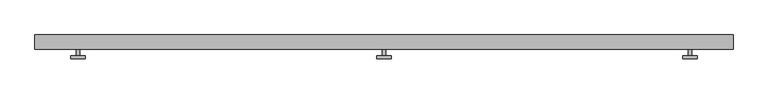
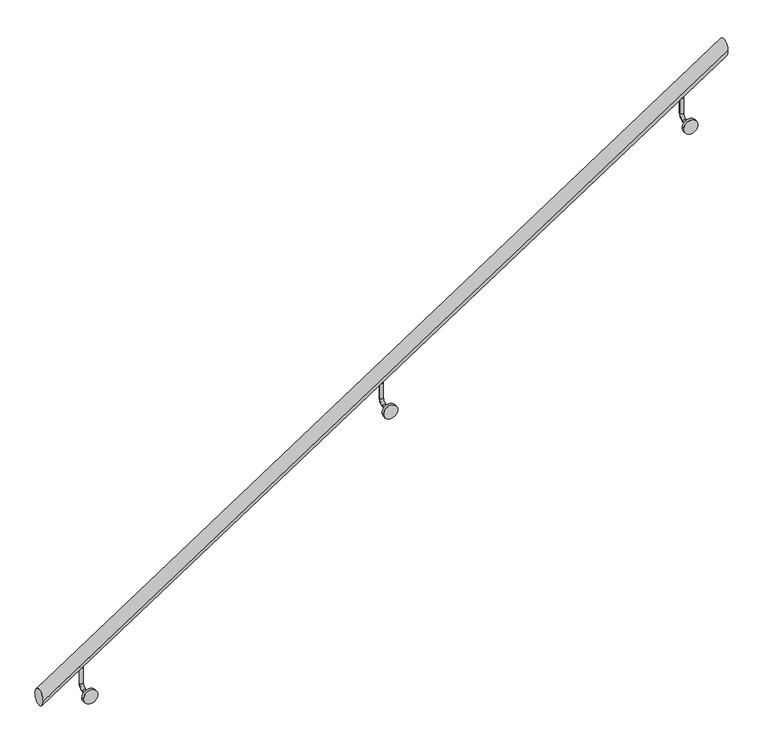
"""IFC4 building model written with IfcOpenShell, lengths in millimetres: railing geometry."""

from ifc_helpers import new_model, si_unit, point, frame, frame_2d, origin, place, context, project, spatial, circle_curve, ellipse_curve, trimmed, segment, composite_curve, outline, extrude, source, transform, mapped, element, save
from ifc_brep_helpers import plane_surface, cylinder_surface, revolved_surface, advanced_brep


def railing_45cfc386(model_context):
    return source(origin(), model_context, "Body", "SolidModel", [
        advanced_brep(
        [(-50271.1127262, 15484.3574868, 2840.3133544), (-50271.1127262, 15434.3574868, 2840.3133544), (-47841.1127262, 15484.3574868, 4430.3133544), (-47841.1127262, 15434.3574868, 4430.3133544)],
        [
            (0, 1, ellipse_curve(frame((-50271.1127262, 15459.3574868, 2840.3133544), z_axis=(-1.0, 0.0, 0.0), x_axis=(0.0, 0.0, -1.0)), 29.8761606, 25.0)),
            (1, 0, ellipse_curve(frame((-50271.1127262, 15459.3574868, 2840.3133544), z_axis=(-1.0, 0.0, 0.0), x_axis=(0.0, 0.0, -1.0)), 29.8761606, 25.0)),
            (2, 3, ellipse_curve(frame((-47841.1127262, 15459.3574868, 4430.3133544), z_axis=(1.0, 0.0, 0.0), x_axis=(0.0, 0.0, -1.0)), 29.8761606, 25.0)),
            (3, 2, ellipse_curve(frame((-47841.1127262, 15459.3574868, 4430.3133544), z_axis=(1.0, 0.0, 0.0), x_axis=(0.0, 0.0, -1.0)), 29.8761606, 25.0)),
            (0, 2),
            (3, 1),
        ],
        [
            plane_surface(frame((-50271.1127262, 15459.3574868, 2870.189515), z_axis=(-1.0, 0.0, 0.0), x_axis=(0.0, 1.0, 0.0))),
            plane_surface(frame((-47841.1127262, 15459.3574868, 4460.189515), z_axis=(1.0, 0.0, 0.0), x_axis=(0.0, 1.0, 0.0))),
            cylinder_surface(frame((-50257.4245344, 15459.3574868, 2849.2698256), z_axis=(-0.8367875758947572, 0.0, -0.547527673116324), x_axis=(0.0, -1.0, 0.0)), 25.0),
        ],
        [
            (0, [[1, 2]]),
            (1, [[3, 4]]),
            (2, [[-1, 5, -4, 6]]),
            (2, [[-2, -6, -3, -5]]),
        ],
    ),
        advanced_brep(
        [(-49062.4627262, 15459.3574868, 3596.139515), (-49049.7627262, 15459.3574868, 3596.139515), (-49062.4627262, 15459.3574868, 3538.989515), (-49049.7627262, 15459.3574868, 3538.989515), (-49049.7627262, 15440.3074868, 3519.939515), (-49062.4627262, 15440.3074868, 3519.939515), (-49062.4627262, 15411.7324868, 3519.939515), (-49049.7627262, 15411.7324868, 3519.939515)],
        [
            (0, 1, circle_curve(frame((-49056.1127262, 15459.3574868, 3596.139515), z_axis=(0.0, 0.0, 1.0), x_axis=(1.0, 0.0, 0.0)), 6.35)),
            (1, 0, circle_curve(frame((-49056.1127262, 15459.3574868, 3596.139515), z_axis=(0.0, 0.0, 1.0), x_axis=(1.0, 0.0, 0.0)), 6.35)),
            (0, 2),
            (2, 3, circle_curve(frame((-49056.1127262, 15459.3574868, 3538.989515), z_axis=(0.0, 0.0, 1.0), x_axis=(1.0, 0.0, 0.0)), 6.35)),
            (3, 1),
            (3, 2, circle_curve(frame((-49056.1127262, 15459.3574868, 3538.989515), z_axis=(0.0, 0.0, 1.0), x_axis=(1.0, 0.0, 0.0)), 6.35)),
            (4, 3, circle_curve(frame((-49049.7627262, 15440.3074868, 3538.989515), z_axis=(1.0, 0.0, 0.0), x_axis=(0.0, 1.0, 0.0)), 19.05)),
            (2, 5, circle_curve(frame((-49062.4627262, 15440.3074868, 3538.989515), z_axis=(-1.0, 0.0, 0.0), x_axis=(0.0, 1.0, 0.0)), 19.05)),
            (5, 4, circle_curve(frame((-49056.1127262, 15440.3074868, 3519.939515), z_axis=(0.0, 1.0, 0.0), x_axis=(1.0, 0.0, 0.0)), 6.35)),
            (4, 5, circle_curve(frame((-49056.1127262, 15440.3074868, 3519.939515), z_axis=(0.0, 1.0, 0.0), x_axis=(1.0, 0.0, 0.0)), 6.35)),
            (6, 7, circle_curve(frame((-49056.1127262, 15411.7324868, 3519.939515), z_axis=(0.0, -1.0, 0.0), x_axis=(1.0, 0.0, 0.0)), 6.35)),
            (7, 6, circle_curve(frame((-49056.1127262, 15411.7324868, 3519.939515), z_axis=(0.0, -1.0, 0.0), x_axis=(1.0, 0.0, 0.0)), 6.35)),
            (5, 6),
            (7, 4),
        ],
        [
            plane_surface(frame((-49049.7627262, 15459.3574868, 3596.139515), z_axis=(0.0, 0.0, 1.0), x_axis=(0.0, -1.0, 0.0))),
            cylinder_surface(frame((-49056.1127262, 15459.3574868, 3596.139515), z_axis=(0.0, 0.0, 1.0), x_axis=(1.0, 0.0, 0.0)), 6.35),
            revolved_surface(trimmed(ellipse_curve(frame((-49056.1127262, 15459.3574868, 3538.989515), z_axis=(0.0, 0.0, 1.0), x_axis=(1.0, 0.0, 0.0)), 6.35, 6.35), [point((-49062.4627262, 15459.3574868, 3538.989515))], [point((-49049.7627262, 15459.3574868, 3538.989515))], True, "CARTESIAN"), (-49056.1127262, 15440.3074868, 3538.989515), (-1.0, 0.0, 0.0)),
            revolved_surface(trimmed(ellipse_curve(frame((-49056.1127262, 15459.3574868, 3538.989515), z_axis=(0.0, 0.0, 1.0), x_axis=(1.0, 0.0, 0.0)), 6.35, 6.35), [point((-49049.7627262, 15459.3574868, 3538.989515))], [point((-49062.4627262, 15459.3574868, 3538.989515))], True, "CARTESIAN"), (-49056.1127262, 15440.3074868, 3538.989515), (-1.0, 0.0, 0.0)),
            plane_surface(frame((-49056.1127262, 15411.7324868, 3513.589515), z_axis=(0.0, -1.0, 0.0), x_axis=(1.0, 0.0, 0.0))),
            cylinder_surface(frame((-49056.1127262, 15440.3074868, 3519.939515), z_axis=(0.0, 1.0, 0.0), x_axis=(1.0, 0.0, 0.0)), 6.35),
        ],
        [
            (0, [[1, 2]]),
            (1, [[-1, 3, 4, 5]]),
            (1, [[-2, -5, 6, -3]]),
            (2, [[7, -4, 8, 9]]),
            (3, [[-8, -6, -7, 10]]),
            (4, [[11, 12]]),
            (5, [[-9, 13, -12, 14]]),
            (5, [[-10, -14, -11, -13]]),
        ],
    ),
        extrude(outline(composite_curve([segment(trimmed(circle_curve(frame_2d((3519.939515, -49056.1127262)), 25.4), [point((3519.939515, -49030.7127262))], [point((3519.939515, -49081.5127262))], False, "CARTESIAN"), True, "CONTINUOUS"), segment(trimmed(circle_curve(frame_2d((3519.939515, -49056.1127262)), 25.4), [point((3519.939515, -49081.5127262))], [point((3519.939515, -49030.7127262))], False, "CARTESIAN"), True, "CONTINUOUS")], self_intersect=False)), frame((0.0, 15402.2074868, 0.0), z_axis=(0.0, 1.0, 0.0), x_axis=(0.0, 0.0, 1.0)), (0.0, 0.0, 1.0), 9.525),
        advanced_brep(
        [(-47997.4627262, 15459.3574868, 4292.9913669), (-47984.7627262, 15459.3574868, 4292.9913669), (-47997.4627262, 15459.3574868, 4235.8413669), (-47984.7627262, 15459.3574868, 4235.8413669), (-47984.7627262, 15440.3074868, 4216.7913669), (-47997.4627262, 15440.3074868, 4216.7913669), (-47997.4627262, 15411.7324868, 4216.7913669), (-47984.7627262, 15411.7324868, 4216.7913669)],
        [
            (0, 1, circle_curve(frame((-47991.1127262, 15459.3574868, 4292.9913669), z_axis=(0.0, 0.0, 1.0), x_axis=(1.0, 0.0, 0.0)), 6.35)),
            (1, 0, circle_curve(frame((-47991.1127262, 15459.3574868, 4292.9913669), z_axis=(0.0, 0.0, 1.0), x_axis=(1.0, 0.0, 0.0)), 6.35)),
            (0, 2),
            (2, 3, circle_curve(frame((-47991.1127262, 15459.3574868, 4235.8413669), z_axis=(0.0, 0.0, 1.0), x_axis=(1.0, 0.0, 0.0)), 6.35)),
            (3, 1),
            (3, 2, circle_curve(frame((-47991.1127262, 15459.3574868, 4235.8413669), z_axis=(0.0, 0.0, 1.0), x_axis=(1.0, 0.0, 0.0)), 6.35)),
            (4, 3, circle_curve(frame((-47984.7627262, 15440.3074868, 4235.8413669), z_axis=(1.0, 0.0, 0.0), x_axis=(0.0, 1.0, 0.0)), 19.05)),
            (2, 5, circle_curve(frame((-47997.4627262, 15440.3074868, 4235.8413669), z_axis=(-1.0, 0.0, 0.0), x_axis=(0.0, 1.0, 0.0)), 19.05)),
            (5, 4, circle_curve(frame((-47991.1127262, 15440.3074868, 4216.7913669), z_axis=(0.0, 1.0, 0.0), x_axis=(1.0, 0.0, 0.0)), 6.35)),
            (4, 5, circle_curve(frame((-47991.1127262, 15440.3074868, 4216.7913669), z_axis=(0.0, 1.0, 0.0), x_axis=(1.0, 0.0, 0.0)), 6.35)),
            (6, 7, circle_curve(frame((-47991.1127262, 15411.7324868, 4216.7913669), z_axis=(0.0, -1.0, 0.0), x_axis=(1.0, 0.0, 0.0)), 6.35)),
            (7, 6, circle_curve(frame((-47991.1127262, 15411.7324868, 4216.7913669), z_axis=(0.0, -1.0, 0.0), x_axis=(1.0, 0.0, 0.0)), 6.35)),
            (5, 6),
            (7, 4),
        ],
        [
            plane_surface(frame((-47984.7627262, 15459.3574868, 4292.9913669), z_axis=(0.0, 0.0, 1.0), x_axis=(0.0, -1.0, 0.0))),
            cylinder_surface(frame((-47991.1127262, 15459.3574868, 4292.9913669), z_axis=(0.0, 0.0, 1.0), x_axis=(1.0, 0.0, 0.0)), 6.35),
            revolved_surface(trimmed(ellipse_curve(frame((-47991.1127262, 15459.3574868, 4235.8413669), z_axis=(0.0, 0.0, 1.0), x_axis=(1.0, 0.0, 0.0)), 6.35, 6.35), [point((-47997.4627262, 15459.3574868, 4235.8413669))], [point((-47984.7627262, 15459.3574868, 4235.8413669))], True, "CARTESIAN"), (-47991.1127262, 15440.3074868, 4235.8413669), (-1.0, 0.0, 0.0)),
            revolved_surface(trimmed(ellipse_curve(frame((-47991.1127262, 15459.3574868, 4235.8413669), z_axis=(0.0, 0.0, 1.0), x_axis=(1.0, 0.0, 0.0)), 6.35, 6.35), [point((-47984.7627262, 15459.3574868, 4235.8413669))], [point((-47997.4627262, 15459.3574868, 4235.8413669))], True, "CARTESIAN"), (-47991.1127262, 15440.3074868, 4235.8413669), (-1.0, 0.0, 0.0)),
            plane_surface(frame((-47991.1127262, 15411.7324868, 4210.4413669), z_axis=(0.0, -1.0, 0.0), x_axis=(1.0, 0.0, 0.0))),
            cylinder_surface(frame((-47991.1127262, 15440.3074868, 4216.7913669), z_axis=(0.0, 1.0, 0.0), x_axis=(1.0, 0.0, 0.0)), 6.35),
        ],
        [
            (0, [[1, 2]]),
            (1, [[-1, 3, 4, 5]]),
            (1, [[-2, -5, 6, -3]]),
            (2, [[7, -4, 8, 9]]),
            (3, [[-8, -6, -7, 10]]),
            (4, [[11, 12]]),
            (5, [[-9, 13, -12, 14]]),
            (5, [[-10, -14, -11, -13]]),
        ],
    ),
        extrude(outline(composite_curve([segment(trimmed(circle_curve(frame_2d((4216.7913669, -47991.1127262)), 25.4), [point((4216.7913669, -47965.7127262))], [point((4216.7913669, -48016.5127262))], False, "CARTESIAN"), True, "CONTINUOUS"), segment(trimmed(circle_curve(frame_2d((4216.7913669, -47991.1127262)), 25.4), [point((4216.7913669, -48016.5127262))], [point((4216.7913669, -47965.7127262))], False, "CARTESIAN"), True, "CONTINUOUS")], self_intersect=False)), frame((0.0, 15402.2074868, 0.0), z_axis=(0.0, 1.0, 0.0), x_axis=(0.0, 0.0, 1.0)), (0.0, 0.0, 1.0), 9.525),
        advanced_brep(
        [(-50127.4627262, 15459.3574868, 2899.2876632), (-50114.7627262, 15459.3574868, 2899.2876632), (-50127.4627262, 15459.3574868, 2842.1376632), (-50114.7627262, 15459.3574868, 2842.1376632), (-50114.7627262, 15440.3074868, 2823.0876632), (-50127.4627262, 15440.3074868, 2823.0876632), (-50127.4627262, 15411.7324868, 2823.0876632), (-50114.7627262, 15411.7324868, 2823.0876632)],
        [
            (0, 1, circle_curve(frame((-50121.1127262, 15459.3574868, 2899.2876632), z_axis=(0.0, 0.0, 1.0), x_axis=(1.0, 0.0, 0.0)), 6.35)),
            (1, 0, circle_curve(frame((-50121.1127262, 15459.3574868, 2899.2876632), z_axis=(0.0, 0.0, 1.0), x_axis=(1.0, 0.0, 0.0)), 6.35)),
            (0, 2),
            (2, 3, circle_curve(frame((-50121.1127262, 15459.3574868, 2842.1376632), z_axis=(0.0, 0.0, 1.0), x_axis=(1.0, 0.0, 0.0)), 6.35)),
            (3, 1),
            (3, 2, circle_curve(frame((-50121.1127262, 15459.3574868, 2842.1376632), z_axis=(0.0, 0.0, 1.0), x_axis=(1.0, 0.0, 0.0)), 6.35)),
            (4, 3, circle_curve(frame((-50114.7627262, 15440.3074868, 2842.1376632), z_axis=(1.0, 0.0, 0.0), x_axis=(0.0, 1.0, 0.0)), 19.05)),
            (2, 5, circle_curve(frame((-50127.4627262, 15440.3074868, 2842.1376632), z_axis=(-1.0, 0.0, 0.0), x_axis=(0.0, 1.0, 0.0)), 19.05)),
            (5, 4, circle_curve(frame((-50121.1127262, 15440.3074868, 2823.0876632), z_axis=(0.0, 1.0, 0.0), x_axis=(1.0, 0.0, 0.0)), 6.35)),
            (4, 5, circle_curve(frame((-50121.1127262, 15440.3074868, 2823.0876632), z_axis=(0.0, 1.0, 0.0), x_axis=(1.0, 0.0, 0.0)), 6.35)),
            (6, 7, circle_curve(frame((-50121.1127262, 15411.7324868, 2823.0876632), z_axis=(0.0, -1.0, 0.0), x_axis=(1.0, 0.0, 0.0)), 6.35)),
            (7, 6, circle_curve(frame((-50121.1127262, 15411.7324868, 2823.0876632), z_axis=(0.0, -1.0, 0.0), x_axis=(1.0, 0.0, 0.0)), 6.35)),
            (5, 6),
            (7, 4),
        ],
        [
            plane_surface(frame((-50114.7627262, 15459.3574868, 2899.2876632), z_axis=(0.0, 0.0, 1.0), x_axis=(0.0, -1.0, 0.0))),
            cylinder_surface(frame((-50121.1127262, 15459.3574868, 2899.2876632), z_axis=(0.0, 0.0, 1.0), x_axis=(1.0, 0.0, 0.0)), 6.35),
            revolved_surface(trimmed(ellipse_curve(frame((-50121.1127262, 15459.3574868, 2842.1376632), z_axis=(0.0, 0.0, 1.0), x_axis=(1.0, 0.0, 0.0)), 6.35, 6.35), [point((-50127.4627262, 15459.3574868, 2842.1376632))], [point((-50114.7627262, 15459.3574868, 2842.1376632))], True, "CARTESIAN"), (-50121.1127262, 15440.3074868, 2842.1376632), (-1.0, 0.0, 0.0)),
            revolved_surface(trimmed(ellipse_curve(frame((-50121.1127262, 15459.3574868, 2842.1376632), z_axis=(0.0, 0.0, 1.0), x_axis=(1.0, 0.0, 0.0)), 6.35, 6.35), [point((-50114.7627262, 15459.3574868, 2842.1376632))], [point((-50127.4627262, 15459.3574868, 2842.1376632))], True, "CARTESIAN"), (-50121.1127262, 15440.3074868, 2842.1376632), (-1.0, 0.0, 0.0)),
            plane_surface(frame((-50121.1127262, 15411.7324868, 2816.7376632), z_axis=(0.0, -1.0, 0.0), x_axis=(1.0, 0.0, 0.0))),
            cylinder_surface(frame((-50121.1127262, 15440.3074868, 2823.0876632), z_axis=(0.0, 1.0, 0.0), x_axis=(1.0, 0.0, 0.0)), 6.35),
        ],
        [
            (0, [[1, 2]]),
            (1, [[-1, 3, 4, 5]]),
            (1, [[-2, -5, 6, -3]]),
            (2, [[7, -4, 8, 9]]),
            (3, [[-8, -6, -7, 10]]),
            (4, [[11, 12]]),
            (5, [[-9, 13, -12, 14]]),
            (5, [[-10, -14, -11, -13]]),
        ],
    ),
        extrude(outline(composite_curve([segment(trimmed(circle_curve(frame_2d((2823.0876632, -50121.1127262)), 25.4), [point((2823.0876632, -50095.7127262))], [point((2823.0876632, -50146.5127262))], False, "CARTESIAN"), True, "CONTINUOUS"), segment(trimmed(circle_curve(frame_2d((2823.0876632, -50121.1127262)), 25.4), [point((2823.0876632, -50146.5127262))], [point((2823.0876632, -50095.7127262))], False, "CARTESIAN"), True, "CONTINUOUS")], self_intersect=False)), frame((0.0, 15402.2074868, 0.0), z_axis=(0.0, 1.0, 0.0), x_axis=(0.0, 0.0, 1.0)), (0.0, 0.0, 1.0), 9.525),
    ])


if __name__ == "__main__":
    model = new_model("IFC4")
    model_context = context("Model", 3, world=origin())
    ifc_project = project(units=[si_unit("LENGTHUNIT", "METRE", prefix="MILLI")], contexts=[model_context])
    site = spatial("IfcSite", under=ifc_project)
    building = spatial("IfcBuilding", under=site)
    placement = place(None, origin())
    railing_shape = railing_45cfc386(model_context)
    element("IfcRailing", 1, at=placement, inside=building, context=model_context, shape_type="MappedRepresentation", body=[
        mapped(railing_shape, transform((0.0, 0.0, 0.0), x_axis=(1.0, 0.0, 0.0), y_axis=(0.0, 1.0, 0.0), z_axis=(0.0, 0.0, 1.0))),
    ])
    save(model, "model.ifc")
